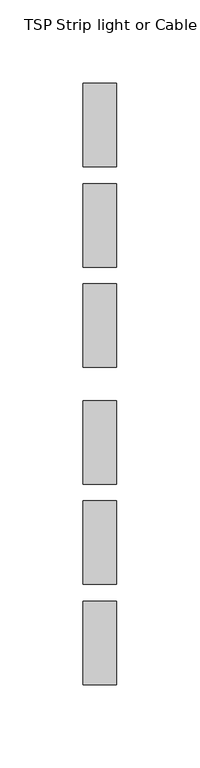
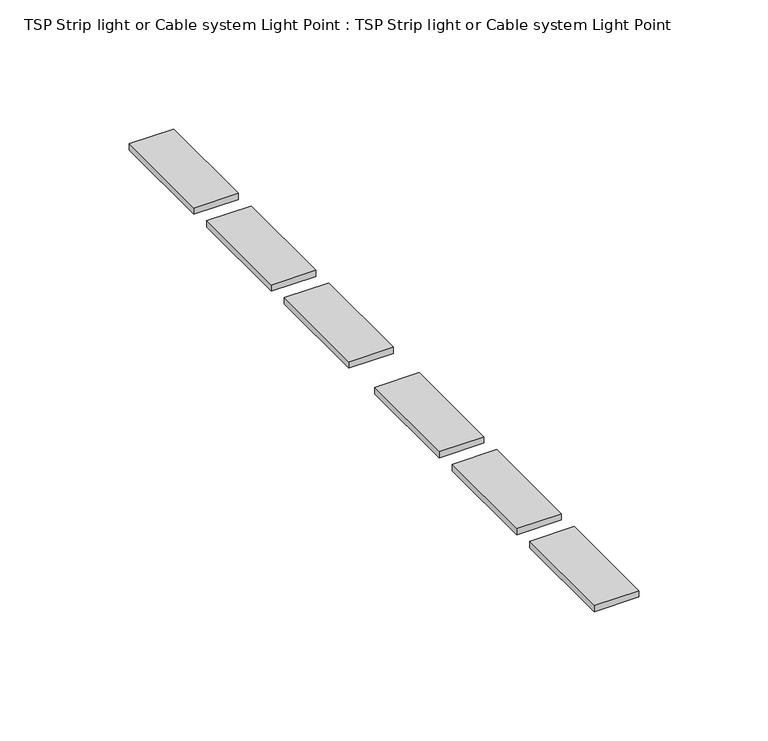
"""IFC4 building model written with IfcOpenShell, lengths in millimetres: proxy geometry, TSP Strip light or Cable system Light Point : TSP Strip light or Cable system Light Point."""

from ifc_helpers import new_model, si_unit, origin, origin_with_axes, place, context, project, spatial, polyline, outline, extrude, source, transform, mapped, element, save


def tsp_strip_light_or_cable_system_light_point_tsp_strip_light_b1916418(model_context):
    return source(origin(), model_context, "Body", "SweptSolid", [
        extrude(outline(polyline([(10.0, 60.0), (10.0, 10.0), (-10.0, 10.0), (-10.0, 60.0), (10.0, 60.0)])), origin_with_axes(), (0.0, 0.0, 1.0), 3.0),
        extrude(outline(polyline([(10.0, 120.0), (10.0, 70.0), (-10.0, 70.0), (-10.0, 120.0), (10.0, 120.0)])), origin_with_axes(), (0.0, 0.0, 1.0), 3.0),
        extrude(outline(polyline([(10.0, 180.0), (10.0, 130.0), (-10.0, 130.0), (-10.0, 180.0), (10.0, 180.0)])), origin_with_axes(), (0.0, 0.0, 1.0), 3.0),
        extrude(outline(polyline([(10.0, -60.0), (-10.0, -60.0), (-10.0, -10.0), (10.0, -10.0), (10.0, -60.0)])), origin_with_axes(), (0.0, 0.0, 1.0), 3.0),
        extrude(outline(polyline([(10.0, -120.0), (-10.0, -120.0), (-10.0, -70.0), (10.0, -70.0), (10.0, -120.0)])), origin_with_axes(), (0.0, 0.0, 1.0), 3.0),
        extrude(outline(polyline([(10.0, -180.0), (-10.0, -180.0), (-10.0, -130.0), (10.0, -130.0), (10.0, -180.0)])), origin_with_axes(), (0.0, 0.0, 1.0), 3.0),
    ])


if __name__ == "__main__":
    model = new_model("IFC4")
    model_context = context("Model", 3, world=origin())
    ifc_project = project(units=[si_unit("LENGTHUNIT", "METRE", prefix="MILLI")], contexts=[model_context])
    site = spatial("IfcSite", under=ifc_project)
    building = spatial("IfcBuilding", under=site)
    placement = place(None, origin())
    tsp_strip_light_or_cable_system_light_point_tsp_strip_light_shape = tsp_strip_light_or_cable_system_light_point_tsp_strip_light_b1916418(model_context)
    element("IfcBuildingElementProxy", 1, Name="TSP Strip light or Cable system Light Point : TSP Strip light or Cable system Light Point", ObjectType="TSP Strip light or Cable system Light Point : TSP Strip light or Cable system Light Point", at=placement, inside=building, context=model_context, shape_type="MappedRepresentation", body=[
        mapped(tsp_strip_light_or_cable_system_light_point_tsp_strip_light_shape, transform((0.0, 0.0, 0.0), x_axis=(1.0, 0.0, 0.0), y_axis=(0.0, 1.0, 0.0), z_axis=(0.0, 0.0, 1.0))),
    ])
    save(model, "model.ifc")

# Revit data of these elements
# Type "TSP Strip light or Cable system Light Point : TSP Strip light or Cable system Light Point"
#   Model = "TSP_ELEC220LEDLP"
#   Default Elevation = 0
# Element 1 (IfcBuildingElementProxy, "TSP Strip light or Cable system Light Point : TSP Strip light or Cable system Light Point")
#   Materials on its faces: "Plastic, Opaque Black"
# Materials
#   "Plastic, Opaque Black": class "Plastic", colour RGB 0 0 0, transparency 0.7, Description = "Plastic, generic, opaque black", Cost = 0
